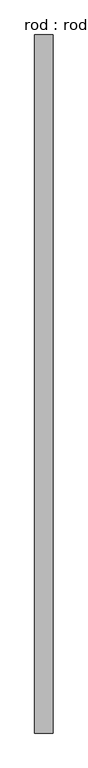
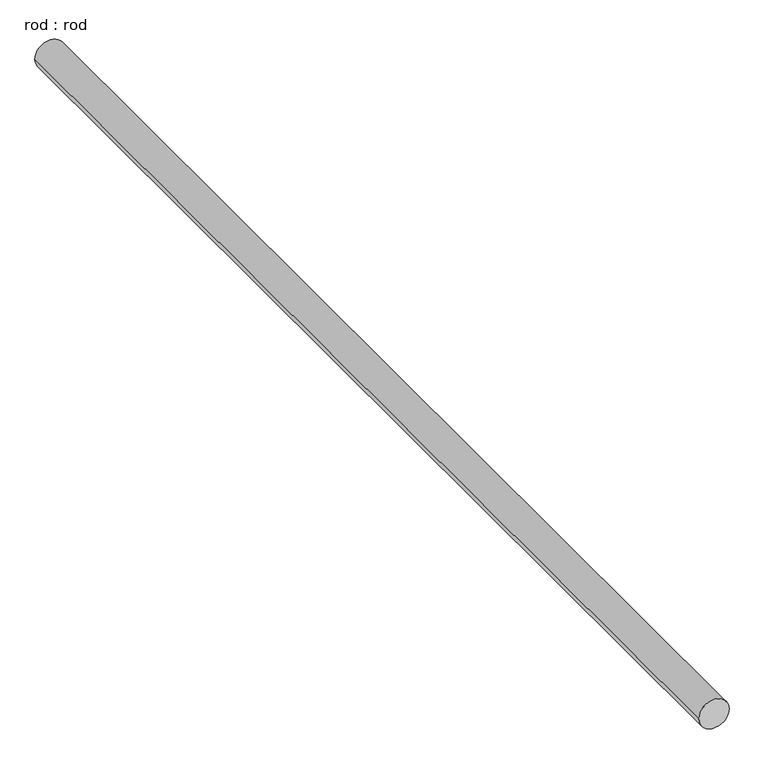
"""IFC4 building model written with IfcOpenShell, lengths in millimetres: proxy geometry, rod : rod."""

from ifc_helpers import new_model, si_unit, point, frame, frame_2d, origin, place, context, project, spatial, circle_curve, trimmed, segment, composite_curve, outline, extrude, source, transform, mapped, element, save


def rod_rod_3e991c1e(model_context):
    return source(origin(), model_context, "Body", "SweptSolid", [
        extrude(outline(composite_curve([segment(trimmed(circle_curve(frame_2d((0.0108462, 0.0)), 200.0), [point((0.0108462, 200.0))], [point((0.0108462, -200.0))], False, "CARTESIAN"), True, "CONTINUOUS"), segment(trimmed(circle_curve(frame_2d((0.0108462, 0.0)), 200.0), [point((0.0108462, -200.0))], [point((0.0108462, 200.0))], False, "CARTESIAN"), True, "CONTINUOUS")], self_intersect=False)), frame((0.0, -3498.2758482, 0.0), z_axis=(0.0, 1.0, 0.0), x_axis=(0.0, 0.0, 1.0)), (0.0, 0.0, 1.0), 15182.0089271),
    ])


if __name__ == "__main__":
    model = new_model("IFC4")
    model_context = context("Model", 3, world=origin())
    ifc_project = project(units=[si_unit("LENGTHUNIT", "METRE", prefix="MILLI")], contexts=[model_context])
    site = spatial("IfcSite", under=ifc_project)
    building = spatial("IfcBuilding", under=site)
    placement = place(None, origin())
    rod_rod_shape = rod_rod_3e991c1e(model_context)
    element("IfcBuildingElementProxy", 1, Name="rod : rod", ObjectType="rod : rod", at=placement, inside=building, context=model_context, shape_type="MappedRepresentation", body=[
        mapped(rod_rod_shape, transform((0.0, 0.0, 0.0), x_axis=(1.0, 0.0, 0.0), y_axis=(0.0, 1.0, 0.0), z_axis=(0.0, 0.0, 1.0))),
    ])
    save(model, "model.ifc")

# Revit data of these elements
# Type "rod : rod"
#   Default Elevation = 0
